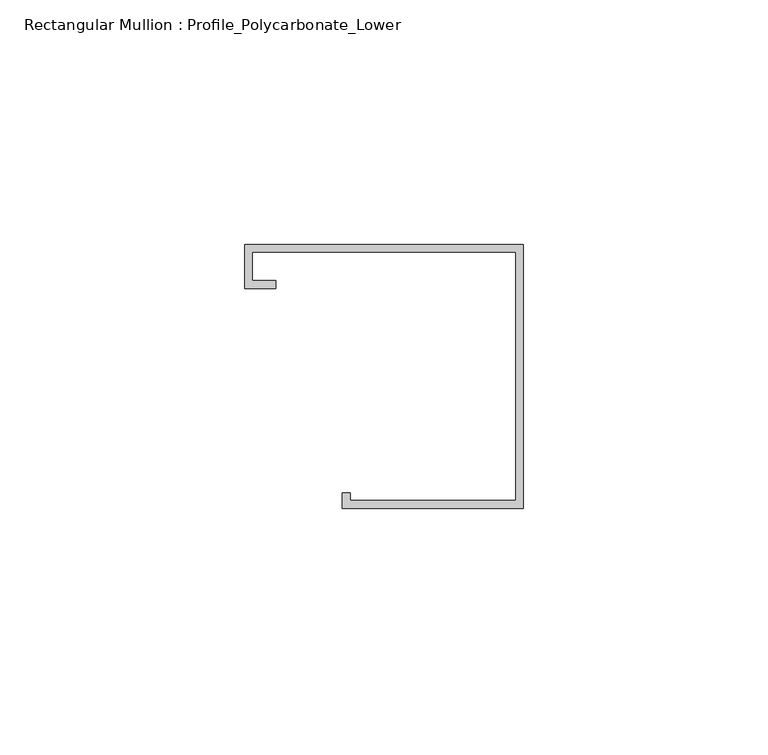
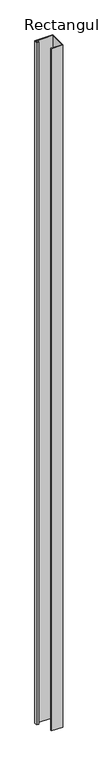
"""IFC4 building model written with IfcOpenShell, lengths in millimetres: member geometry, Rectangular Mullion : Profile_Polycarbonate_Lower."""

from ifc_helpers import new_model, si_unit, frame, origin, place, context, project, spatial, polyline, outline, extrude, source, transform, mapped, element, save


def rectangular_mullion_profile_polycarbonate_lower_3128b5d2(model_context):
    return source(origin(), model_context, "Body", "SweptSolid", [
        extrude(outline(polyline([(0.0, 28.984575), (0.0, -25.015825), (-36.9824, -25.015825), (-36.9824, -21.840825), (-35.3949, -21.840825), (-35.3949, -23.428325), (-1.5875, -23.428325), (-1.5875, 27.397075), (-55.4101, 27.397075), (-55.4101, 21.580475), (-50.6476, 21.580475), (-50.6476, 19.992975), (-56.9976, 19.992975), (-56.9976, 28.984575), (0.0, 28.984575)])), frame((0.0, 0.0, -2273.4524), z_axis=(0.0, 0.0, 1.0), x_axis=(1.0, 0.0, 0.0)), (0.0, 0.0, 1.0), 2273.4524),
    ])


if __name__ == "__main__":
    model = new_model("IFC4")
    model_context = context("Model", 3, world=origin())
    ifc_project = project(units=[si_unit("LENGTHUNIT", "METRE", prefix="MILLI")], contexts=[model_context])
    site = spatial("IfcSite", under=ifc_project)
    building = spatial("IfcBuilding", under=site)
    placement = place(None, origin())
    rectangular_mullion_profile_polycarbonate_lower_shape = rectangular_mullion_profile_polycarbonate_lower_3128b5d2(model_context)
    element("IfcMember", 1, ObjectType="Rectangular Mullion : Profile_Polycarbonate_Lower", at=placement, inside=building, context=model_context, shape_type="MappedRepresentation", body=[
        mapped(rectangular_mullion_profile_polycarbonate_lower_shape, transform((0.0, 0.0, 0.0), x_axis=(1.0, 0.0, 0.0), y_axis=(0.0, 1.0, 0.0), z_axis=(0.0, 0.0, 1.0))),
    ])
    save(model, "model.ifc")

# Revit data of these elements
# Type "Rectangular Mullion : Profile_Polycarbonate_Lower"
#   built-in parameter 1007322 = 0.177167 (stored number, unit not read)
#   built-in parameter 1007321 = 0 (stored number, unit not read)
#   built-in parameter 1007320 = 0.00520833 (stored number, unit not read)
